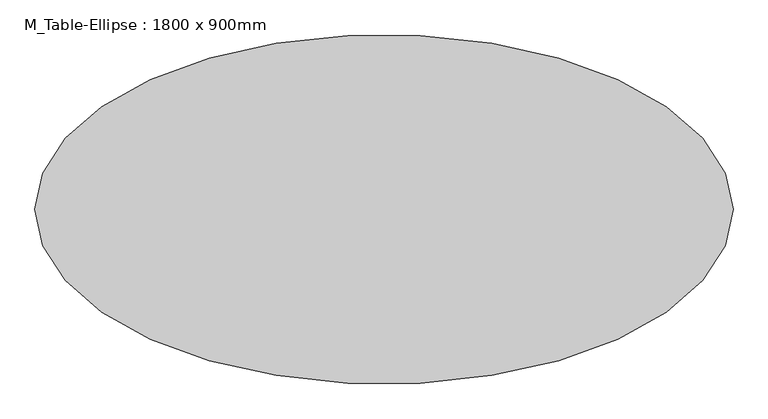
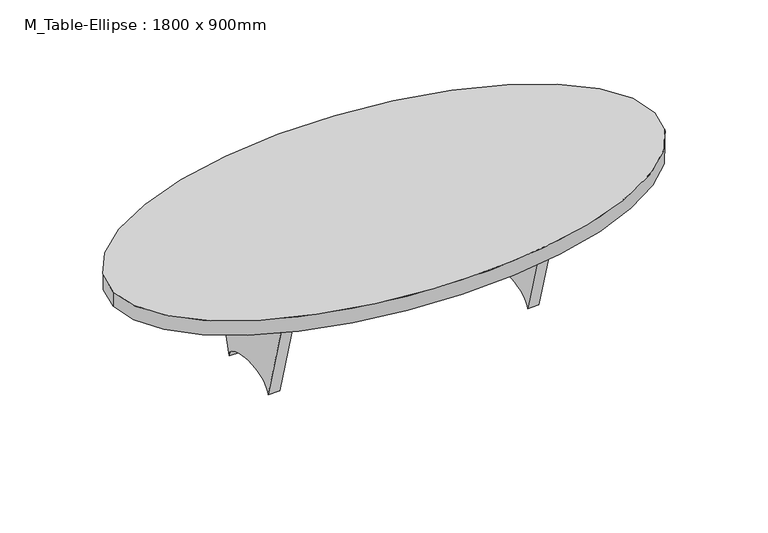
"""IFC4 building model written with IfcOpenShell, lengths in millimetres: furniture geometry, M_Table-Ellipse : 1800 x 900mm."""

from ifc_helpers import new_model, si_unit, point, frame, origin, place, context, project, spatial, ellipse_curve, trimmed, source, transform, mapped, element, save
from ifc_brep_helpers import plane_surface, extruded_surface, advanced_brep


def m_table_ellipse_1800_x_900mm_db041c4c(model_context):
    return source(origin(), model_context, "Body", "AdvancedBrep", [
        advanced_brep(
        [(-411.9, 19.05, 399.2), (411.9, 19.05, 399.2), (411.9, 19.05, 266.1333333), (-411.9, 19.05, 266.1333333), (-411.9, -19.05, 399.2), (-411.9, -19.05, 266.1333333), (411.9, -19.05, 266.1333333), (411.9, -19.05, 399.2)],
        [
            (0, 1),
            (1, 2),
            (2, 3, ellipse_curve(frame((0.0, 19.05, 266.1333333), z_axis=(0.0, -1.0, 0.0), x_axis=(1.0, 0.0, 0.0)), 411.9, 101.6)),
            (3, 0),
            (4, 5),
            (5, 6, ellipse_curve(frame((0.0, -19.05, 266.1333333), z_axis=(0.0, 1.0, 0.0), x_axis=(1.0, 0.0, 0.0)), 411.9, 101.6)),
            (6, 7),
            (7, 4),
            (0, 4),
            (7, 1),
            (6, 2),
            (5, 3),
        ],
        [
            plane_surface(frame((-411.9, 19.05, 399.2), z_axis=(0.0, 1.0, 0.0), x_axis=(1.0, 0.0, 0.0))),
            plane_surface(frame((-411.9, -19.05, 399.2), z_axis=(0.0, -1.0, 0.0), x_axis=(-1.0, 0.0, 0.0))),
            plane_surface(frame((-411.9, 19.05, 399.2), z_axis=(0.0, 0.0, 1.0), x_axis=(0.0, -1.0, 0.0))),
            plane_surface(frame((411.9, 19.05, 399.2), z_axis=(1.0, 0.0, 0.0), x_axis=(0.0, -1.0, 0.0))),
            extruded_surface(trimmed(ellipse_curve(frame((0.0, -57.15, 266.1333333), z_axis=(0.0, -1.0, 0.0), x_axis=(1.0, 0.0, 0.0)), 411.9, 101.6), [point((411.9, -57.15, 266.1333333))], [point((-411.9, -57.15, 266.1333333))], True, "CARTESIAN"), (0.0, 38.099999999999994, 0.0), 38.099999999999994),
            plane_surface(frame((-411.9, 19.05, 266.1333333), z_axis=(-1.0, 0.0, 0.0), x_axis=(0.0, -1.0, 0.0))),
        ],
        [
            (0, [[1, 2, 3, 4]]),
            (1, [[5, 6, 7, 8]]),
            (2, [[-1, 9, -8, 10]]),
            (3, [[-2, -10, -7, 11]]),
            (4, [[-3, -11, -6, 12]]),
            (5, [[-4, -12, -5, -9]]),
        ],
    ),
        advanced_brep(
        [(450.0, 225.0, 399.2), (450.0, -225.0, 399.2), (450.0, -112.5, 0.0), (450.0, 112.5, 0.0), (411.9, 225.0, 399.2), (411.9, 112.5, 0.0), (411.9, -112.5, 0.0), (411.9, -225.0, 399.2)],
        [
            (0, 1),
            (1, 2),
            (2, 3, ellipse_curve(frame((450.0, 0.0, 0.0), z_axis=(-1.0, 0.0, 0.0), x_axis=(0.0, 1.0, 0.0)), 112.5, 50.8)),
            (3, 0),
            (4, 5),
            (5, 6, ellipse_curve(frame((411.9, 0.0, 0.0), z_axis=(1.0, 0.0, 0.0), x_axis=(0.0, 1.0, 0.0)), 112.5, 50.8)),
            (6, 7),
            (7, 4),
            (0, 4),
            (7, 1),
            (6, 2),
            (5, 3),
        ],
        [
            plane_surface(frame((450.0, -225.0, 399.2), z_axis=(1.0, 0.0, 0.0), x_axis=(0.0, -1.0, 0.0))),
            plane_surface(frame((411.9, -225.0, 399.2), z_axis=(-1.0, 0.0, 0.0), x_axis=(0.0, 1.0, 0.0))),
            plane_surface(frame((450.0, 225.0, 399.2), z_axis=(0.0, 0.0, 1.0), x_axis=(-1.0, 0.0, 0.0))),
            plane_surface(frame((450.0, -225.0, 399.2), z_axis=(0.0, -0.962509416119105, -0.2712482698231631), x_axis=(-1.0, 0.0, 0.0))),
            extruded_surface(trimmed(ellipse_curve(frame((373.8, 0.0, 0.0), z_axis=(-1.0, 0.0, 0.0), x_axis=(0.0, 1.0, 0.0)), 112.5, 50.8), [point((373.8, -112.5, 0.0))], [point((373.8, 112.5, 0.0))], True, "CARTESIAN"), (38.099999999999966, 0.0, 0.0), 38.099999999999966),
            plane_surface(frame((450.0, 112.5, 0.0), z_axis=(0.0, 0.9625094161191101, -0.27124826982314537), x_axis=(-1.0, 0.0, 0.0))),
        ],
        [
            (0, [[1, 2, 3, 4]]),
            (1, [[5, 6, 7, 8]]),
            (2, [[-1, 9, -8, 10]]),
            (3, [[-2, -10, -7, 11]]),
            (4, [[-3, -11, -6, 12]]),
            (5, [[-4, -12, -5, -9]]),
        ],
    ),
        advanced_brep(
        [(-411.9, 225.0, 399.2), (-411.9, -225.0, 399.2), (-411.9, -112.5, 0.0), (-411.9, 112.5, 0.0), (-450.0, 225.0, 399.2), (-450.0, 112.5, 0.0), (-450.0, -112.5, 0.0), (-450.0, -225.0, 399.2)],
        [
            (0, 1),
            (1, 2),
            (2, 3, ellipse_curve(frame((-411.9, 0.0, 0.0), z_axis=(-1.0, 0.0, 0.0), x_axis=(0.0, 1.0, 0.0)), 112.5, 50.8)),
            (3, 0),
            (4, 5),
            (5, 6, ellipse_curve(frame((-450.0, 0.0, 0.0), z_axis=(1.0, 0.0, 0.0), x_axis=(0.0, 1.0, 0.0)), 112.5, 50.8)),
            (6, 7),
            (7, 4),
            (0, 4),
            (7, 1),
            (6, 2),
            (5, 3),
        ],
        [
            plane_surface(frame((-411.9, -225.0, 399.2), z_axis=(1.0, 0.0, 0.0), x_axis=(0.0, -1.0, 0.0))),
            plane_surface(frame((-450.0, -225.0, 399.2), z_axis=(-1.0, 0.0, 0.0), x_axis=(0.0, 1.0, 0.0))),
            plane_surface(frame((-411.9, 225.0, 399.2), z_axis=(0.0, 0.0, 1.0), x_axis=(-1.0, 0.0, 0.0))),
            plane_surface(frame((-411.9, -225.0, 399.2), z_axis=(0.0, -0.9625094161191028, -0.27124826982317146), x_axis=(-1.0, 0.0, 0.0))),
            extruded_surface(trimmed(ellipse_curve(frame((-488.1, 0.0, 0.0), z_axis=(-1.0, 0.0, 0.0), x_axis=(0.0, 1.0, 0.0)), 112.5, 50.8), [point((-488.1, -112.5, 0.0))], [point((-488.1, 112.5, 0.0))], True, "CARTESIAN"), (38.10000000000002, 0.0, 0.0), 38.10000000000002),
            plane_surface(frame((-411.9, 112.5, 0.0), z_axis=(0.0, 0.9625094161191071, -0.2712482698231561), x_axis=(-1.0, 0.0, 0.0))),
        ],
        [
            (0, [[1, 2, 3, 4]]),
            (1, [[5, 6, 7, 8]]),
            (2, [[-1, 9, -8, 10]]),
            (3, [[-2, -10, -7, 11]]),
            (4, [[-3, -11, -6, 12]]),
            (5, [[-4, -12, -5, -9]]),
        ],
    ),
        advanced_brep(
        [(-900.0, 0.0, 450.0), (900.0, 0.0, 450.0), (-900.0, 0.0, 399.2), (900.0, 0.0, 399.2)],
        [
            (0, 1, ellipse_curve(frame((0.0, 0.0, 450.0), z_axis=(0.0, 0.0, 1.0), x_axis=(1.0, 0.0, 0.0)), 900.0, 450.0)),
            (1, 0, ellipse_curve(frame((0.0, 0.0, 450.0), z_axis=(0.0, 0.0, 1.0), x_axis=(1.0, 0.0, 0.0)), 900.0, 450.0)),
            (2, 3, ellipse_curve(frame((0.0, 0.0, 399.2), z_axis=(0.0, 0.0, -1.0), x_axis=(1.0, 0.0, 0.0)), 900.0, 450.0)),
            (3, 2, ellipse_curve(frame((0.0, 0.0, 399.2), z_axis=(0.0, 0.0, -1.0), x_axis=(1.0, 0.0, 0.0)), 900.0, 450.0)),
            (0, 2),
            (3, 1),
        ],
        [
            plane_surface(frame((900.0, 0.0, 450.0), z_axis=(0.0, 0.0, 1.0), x_axis=(0.0, 1.0, 0.0))),
            plane_surface(frame((900.0, 0.0, 399.2), z_axis=(0.0, 0.0, -1.0), x_axis=(0.0, -1.0, 0.0))),
            extruded_surface(trimmed(ellipse_curve(frame((0.0, 0.0, 348.4), z_axis=(0.0, 0.0, 1.0), x_axis=(1.0, 0.0, 0.0)), 900.0, 450.0), [point((-900.0, 0.0, 348.4))], [point((900.0, 0.0, 348.4))], True, "CARTESIAN"), (0.0, 0.0, 50.80000000000001), 50.80000000000001),
            extruded_surface(trimmed(ellipse_curve(frame((0.0, 0.0, 348.4), z_axis=(0.0, 0.0, 1.0), x_axis=(1.0, 0.0, 0.0)), 900.0, 450.0), [point((900.0, 0.0, 348.4))], [point((-900.0, 0.0, 348.4))], True, "CARTESIAN"), (0.0, 0.0, 50.80000000000001), 50.80000000000001),
        ],
        [
            (0, [[1, 2]]),
            (1, [[3, 4]]),
            (2, [[-1, 5, -4, 6]]),
            (3, [[-2, -6, -3, -5]]),
        ],
    ),
    ])


if __name__ == "__main__":
    model = new_model("IFC4")
    model_context = context("Model", 3, world=origin())
    ifc_project = project(units=[si_unit("LENGTHUNIT", "METRE", prefix="MILLI")], contexts=[model_context])
    site = spatial("IfcSite", under=ifc_project)
    building = spatial("IfcBuilding", under=site)
    placement = place(None, origin())
    m_table_ellipse_1800_x_900mm_shape = m_table_ellipse_1800_x_900mm_db041c4c(model_context)
    element("IfcFurniture", 1, ObjectType="M_Table-Ellipse : 1800 x 900mm", at=placement, inside=building, context=model_context, shape_type="MappedRepresentation", body=[
        mapped(m_table_ellipse_1800_x_900mm_shape, transform((0.0, 0.0, 0.0), x_axis=(1.0, 0.0, 0.0), y_axis=(0.0, 1.0, 0.0), z_axis=(0.0, 0.0, 1.0))),
    ])
    save(model, "model.ifc")

# Revit data of these elements
# Type "M_Table-Ellipse : 1800 x 900mm"
#   Half Width = 0.45 m
#   Half Length = 0.9 m
#   Height = 0.45 m
#   Length = 1.8 m
#   Width = 0.9 m
#   Base Material = Birch
#   Top Material = Laminate - Black
#   Default Elevation = 0
#   Assembly Code = ""
# Element 1 (IfcFurniture, "M_Table-Ellipse : 1800 x 900mm")
#   Materials on its faces: "Birch", "Laminate - Black"
# Materials
#   "Birch": class "Wood", colour RGB 224 178 126, transparency 0, Description = "Betula Alleghaniensis", Cost = 0
#   "Laminate - Black": class "Miscellaneous", colour RGB 0 0 0, transparency 0
